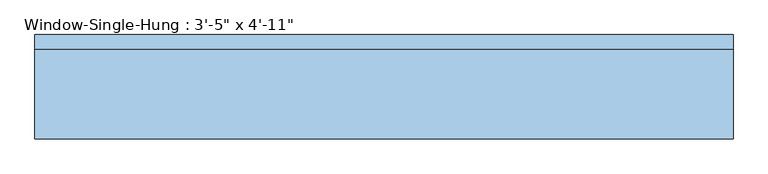
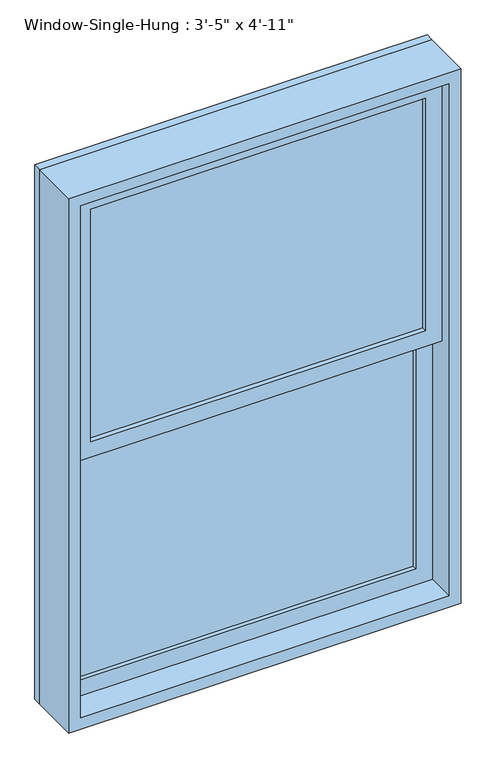
"""IFC4 building model written with IfcOpenShell, lengths in millimetres: window geometry."""

import ifcopenshell
import ifcopenshell.guid

model = None  # the IFC model being written
_history = None  # IfcOwnerHistory: only IFC2X3 demands one
_inside = {}  # id of a spatial element -> (the spatial element, [elements in it])
_under = {}  # id of a project, library or spatial element -> (it, [spatial elements below it])
_declared = {}  # id of a project -> (the project, [libraries it declares])
_typed = {}  # id of a type object -> (the type object, [elements of that type])
_made_of = {}  # id of a material, layer set ... -> (it, [elements and type objects made of it])


def new_model(schema):
    """Start an empty IFC model of exactly this schema.

    Asked for "IFC4X3", IfcOpenShell would pick the latest addendum, in which some entities
    have other attributes; the version numbers below select the first issue.
    IFC2X3 requires an IfcOwnerHistory on every rooted entity: one is made here for all.
    """
    global model, _history
    if schema == "IFC4X3":
        model = ifcopenshell.file(schema_version=(4, 3, 0, 0))
    else:
        model = ifcopenshell.file(schema=schema)
    _inside.clear()
    _under.clear()
    _declared.clear()
    _typed.clear()
    _made_of.clear()
    _history = None
    if model.schema == "IFC2X3":
        org = make("IfcOrganization", Name="unknown")
        user = make(
            "IfcPersonAndOrganization",
            ThePerson=make("IfcPerson", FamilyName="unknown"),
            TheOrganization=org,
        )
        app = make(
            "IfcApplication",
            ApplicationDeveloper=org,
            Version="unknown",
            ApplicationFullName="unknown",
            ApplicationIdentifier="unknown",
        )
        _history = make(
            "IfcOwnerHistory",
            OwningUser=user,
            OwningApplication=app,
            ChangeAction="ADDED",
            CreationDate=0,
        )
    return model


def make(cls, **values):
    """One entity of the class cls with the attributes given. An attribute that is None is left unset."""
    return model.create_entity(
        cls, **{name: value for name, value in values.items() if value is not None}
    )


def rooted(cls, **values):
    """An entity with a GlobalId (a new one), such as an element, a storey or a relation."""
    return make(cls, GlobalId=ifcopenshell.guid.new(), OwnerHistory=_history, **values)


def si_unit(unit_type, name, prefix=None):
    """IfcSIUnit, for example si_unit("LENGTHUNIT", "METRE", prefix="MILLI")."""
    return make("IfcSIUnit", UnitType=unit_type, Prefix=prefix, Name=name)


def assignment(units):
    """IfcUnitAssignment: the units of a project."""
    return None if units is None else make("IfcUnitAssignment", Units=units)


def point(xyz):
    """IfcCartesianPoint."""
    return None if xyz is None else make("IfcCartesianPoint", Coordinates=xyz)


def direction(xyz):
    """IfcDirection."""
    return None if xyz is None else make("IfcDirection", DirectionRatios=xyz)


def frame(location, z_axis=None, x_axis=None):
    """IfcAxis2Placement3D, a coordinate frame: its origin and axes. An axis left out is left unset."""
    return make(
        "IfcAxis2Placement3D",
        Location=point(location),
        Axis=direction(z_axis),
        RefDirection=direction(x_axis),
    )


def origin():
    """The frame at (0, 0, 0) with its axes left unset."""
    return frame((0.0, 0.0, 0.0))


def place(relative_to, where):
    """IfcLocalPlacement: puts the frame where relative to a parent placement (None: the world)."""
    return make(
        "IfcLocalPlacement", PlacementRelTo=relative_to, RelativePlacement=where
    )


def context(
    kind, dimensions, precision=None, world=None, true_north=None, identifier=None
):
    """IfcGeometricRepresentationContext, for example the 3D "Model" context."""
    return make(
        "IfcGeometricRepresentationContext",
        ContextIdentifier=identifier,
        ContextType=kind,
        CoordinateSpaceDimension=dimensions,
        Precision=precision,
        WorldCoordinateSystem=world,
        TrueNorth=true_north,
    )


def project(units=None, contexts=None):
    """IfcProject with its units and contexts."""
    return rooted(
        "IfcProject",
        Name="project",
        RepresentationContexts=contexts,
        UnitsInContext=assignment(units),
    )


def spatial(cls, under=None, at=None, **own):
    """A site, building, storey or space (cls), placed at a placement, below another one or the project."""
    s = rooted(cls, ObjectPlacement=at, **own)
    if under is not None:
        _under.setdefault(under.id(), (under, []))[1].append(s)
    return s


def polyline(points):
    """IfcPolyline through the points."""
    return make("IfcPolyline", Points=[point(p) for p in points])


def outline(outer, holes=None, kind="AREA"):
    """IfcArbitraryClosedProfileDef: a profile drawn as a closed curve; with holes, ...WithVoids."""
    if holes is None:
        return make("IfcArbitraryClosedProfileDef", ProfileType=kind, OuterCurve=outer)
    return make(
        "IfcArbitraryProfileDefWithVoids",
        ProfileType=kind,
        OuterCurve=outer,
        InnerCurves=holes,
    )


def extrude(swept, where, along, depth):
    """IfcExtrudedAreaSolid: the profile swept, set in the frame where, extruded along a direction by depth."""
    return make(
        "IfcExtrudedAreaSolid",
        SweptArea=swept,
        Position=where,
        ExtrudedDirection=direction(along),
        Depth=depth,
    )


def shape(context_of_items, identifier, shape_type, items):
    """IfcShapeRepresentation: the items that make up one representation, for example the "Body"."""
    return make(
        "IfcShapeRepresentation",
        ContextOfItems=context_of_items,
        RepresentationIdentifier=identifier,
        RepresentationType=shape_type,
        Items=items,
    )


def source(mapping_origin, context_of_items, identifier, shape_type, items):
    """IfcRepresentationMap: a shape defined once, which mapped items show again and again."""
    return make(
        "IfcRepresentationMap",
        MappingOrigin=mapping_origin,
        MappedRepresentation=shape(context_of_items, identifier, shape_type, items),
    )


def transform(
    local_origin,
    x_axis=None,
    y_axis=None,
    z_axis=None,
    scale=None,
    scale2=None,
    scale3=None,
    uniform=True,
):
    """IfcCartesianTransformationOperator3D, or its non-uniform kind. x_axis, y_axis, z_axis: its Axis1, 2, 3."""
    if uniform:
        return make(
            "IfcCartesianTransformationOperator3D",
            Axis1=direction(x_axis),
            Axis2=direction(y_axis),
            LocalOrigin=point(local_origin),
            Scale=scale,
            Axis3=direction(z_axis),
        )
    return make(
        "IfcCartesianTransformationOperator3DnonUniform",
        Axis1=direction(x_axis),
        Axis2=direction(y_axis),
        LocalOrigin=point(local_origin),
        Scale=scale,
        Axis3=direction(z_axis),
        Scale2=scale2,
        Scale3=scale3,
    )


def mapped(mapping_source, mapping_target):
    """IfcMappedItem: shows the shape of a source again, moved by a transform."""
    return make(
        "IfcMappedItem", MappingSource=mapping_source, MappingTarget=mapping_target
    )


def made_of(thing, what):
    """Note that an element or type object is made of a material, layer set ...; save() writes the relation."""
    if what is not None:
        _made_of.setdefault(what.id(), (what, []))[1].append(thing)
    return thing


def element(
    cls,
    number,
    at=None,
    inside=None,
    cuts=None,
    type_object=None,
    material=None,
    context=None,
    identifier="Body",
    shape_type=None,
    held_by="IfcProductDefinitionShape",
    body=None,
    shapes=None,
    **own,
):
    """One element of the class cls, such as IfcWall. Its Tag is "e" and its number.

    at: its placement. inside: the storey or other place that contains it. cuts: it is an
    opening in that element (IfcRelVoidsElement). A single representation is given by context,
    identifier, shape_type and body (its items); several are given by shapes. held_by: the class
    of the entity that holds the representations. save() writes the other relations.
    """
    e = rooted(cls, Tag="e%d" % number, ObjectPlacement=at, **own)
    if body is not None:
        shapes = [shape(context, identifier, shape_type, body)]
    if shapes is not None:
        e.Representation = make(held_by, Representations=shapes)
    if inside is not None:
        _inside.setdefault(inside.id(), (inside, []))[1].append(e)
    if cuts is not None:
        rooted(
            "IfcRelVoidsElement", RelatingBuildingElement=cuts, RelatedOpeningElement=e
        )
    if type_object is not None:
        _typed.setdefault(type_object.id(), (type_object, []))[1].append(e)
    return made_of(e, material)


def aggregate(whole, parts):
    """IfcRelAggregates: a whole, such as a stair, and the parts it consists of."""
    return rooted("IfcRelAggregates", RelatingObject=whole, RelatedObjects=parts)


def save(model, path):
    """Write the relations noted so far, then the file.

    IfcRelAggregates (storeys below a building ...), IfcRelContainedInSpatialStructure (elements
    in a storey), IfcRelDefinesByType, IfcRelAssociatesMaterial and IfcRelDeclares: one each for
    every whole, place, type object, material and project.
    """
    for whole, parts in _under.values():
        aggregate(whole, parts)
    for where, things in _inside.values():
        rooted(
            "IfcRelContainedInSpatialStructure",
            RelatedElements=things,
            RelatingStructure=where,
        )
    for kind, things in _typed.values():
        rooted("IfcRelDefinesByType", RelatedObjects=things, RelatingType=kind)
    for what, things in _made_of.values():
        rooted("IfcRelAssociatesMaterial", RelatedObjects=things, RelatingMaterial=what)
    for by, libraries in _declared.values():
        rooted("IfcRelDeclares", RelatingContext=by, RelatedDefinitions=libraries)
    model.write(path)


def window_d73c3647(model_context):
    return source(origin(), model_context, "Body", "SweptSolid", [
        extrude(outline(polyline([(444.5, 1.5875), (-444.5, 1.5875), (-444.5, 7.9375), (444.5, 7.9375), (444.5, 1.5875)])), frame((0.0, 0.0, 990.6), z_axis=(0.0, 0.0, 1.0), x_axis=(1.0, 0.0, 0.0)), (0.0, 0.0, 1.0), 650.875),
        extrude(outline(polyline([(-444.5, 14.2875), (-444.5, 20.6375), (444.5, 20.6375), (444.5, 14.2875), (-444.5, 14.2875)])), frame((0.0, 0.0, 990.6), z_axis=(0.0, 0.0, 1.0), x_axis=(1.0, 0.0, 0.0)), (0.0, 0.0, 1.0), 650.875),
        extrude(outline(polyline([(444.5, -42.8625), (-444.5, -42.8625), (-444.5, -36.5125), (444.5, -36.5125), (444.5, -42.8625)])), frame((0.0, 0.0, 1685.925), z_axis=(0.0, 0.0, 1.0), x_axis=(1.0, 0.0, 0.0)), (0.0, 0.0, 1.0), 650.875),
        extrude(outline(polyline([(-444.5, -30.1625), (-444.5, -23.8125), (444.5, -23.8125), (444.5, -30.1625), (-444.5, -30.1625)])), frame((0.0, 0.0, 1685.925), z_axis=(0.0, 0.0, 1.0), x_axis=(1.0, 0.0, 0.0)), (0.0, 0.0, 1.0), 650.875),
        extrude(outline(polyline([(1685.925, 488.95), (1685.925, -488.95), (946.15, -488.95), (946.15, 488.95), (1685.925, 488.95)]), holes=[polyline([(1641.475, -444.5), (1641.475, 444.5), (990.6, 444.5), (990.6, -444.5), (1641.475, -444.5)])]), frame((0.0, -11.1125, 0.0), z_axis=(0.0, 1.0, 0.0), x_axis=(0.0, 0.0, 1.0)), (0.0, 0.0, 1.0), 44.45),
        extrude(outline(polyline([(2381.25, 488.95), (2381.25, -488.95), (1641.475, -488.95), (1641.475, 488.95), (2381.25, 488.95)]), holes=[polyline([(2336.8, -444.5), (2336.8, 444.5), (1685.925, 444.5), (1685.925, -444.5), (2336.8, -444.5)])]), frame((0.0, -55.5625, 0.0), z_axis=(0.0, 1.0, 0.0), x_axis=(0.0, 0.0, 1.0)), (0.0, 0.0, 1.0), 44.45),
        extrude(outline(polyline([(2413.0, 520.7), (2413.0, -520.7), (914.4, -520.7), (914.4, 520.7), (2413.0, 520.7)]), holes=[polyline([(2381.25, -488.95), (2381.25, 488.95), (946.15, 488.95), (946.15, -488.95), (2381.25, -488.95)])]), frame((0.0, -87.3125, 0.0), z_axis=(0.0, 1.0, 0.0), x_axis=(0.0, 0.0, 1.0)), (0.0, 0.0, 1.0), 133.35),
        extrude(outline(polyline([(2413.0, 520.7), (2413.0, -520.7), (914.4, -520.7), (914.4, 520.7), (2413.0, 520.7)]), holes=[polyline([(2393.95, 501.65), (933.45, 501.65), (933.45, -501.65), (2393.95, -501.65), (2393.95, 501.65)])]), frame((0.0, 46.0375, 0.0), z_axis=(0.0, 1.0, 0.0), x_axis=(0.0, 0.0, 1.0)), (0.0, 0.0, 1.0), 22.225),
    ])


if __name__ == "__main__":
    model = new_model("IFC4")
    model_context = context("Model", 3, world=origin())
    ifc_project = project(units=[si_unit("LENGTHUNIT", "METRE", prefix="MILLI")], contexts=[model_context])
    site = spatial("IfcSite", under=ifc_project)
    building = spatial("IfcBuilding", under=site)
    placement = place(None, origin())
    window_shape = window_d73c3647(model_context)
    element("IfcWindow", 1, ObjectType="Window-Single-Hung : 3'-5\" x 4'-11\"", at=placement, inside=building, context=model_context, shape_type="MappedRepresentation", body=[
        mapped(window_shape, transform((0.0, 0.0, 0.0), x_axis=(1.0, 0.0, 0.0), y_axis=(0.0, 1.0, 0.0), z_axis=(0.0, 0.0, 1.0))),
    ])
    save(model, "model.ifc")

# Revit data of these elements
# Type "Window-Single-Hung : 3'-5\" x 4'-11\""
#   Type Mark = "21"
#   Fire Rating = "0.5h"
#   Construction Type Id = "DG-DR"
#   Assembly Code = "B2020100"
#   Analytic Construction = "Double glazing - domestic"
#   Wall Thickness [instance default] = 0' - 6"
#   Window Inset [instance default] = 0' - 0"
#   Visual Light Transmittance = 0.81
#   Thermal Resistance (R) = 0.319569 (m²·K)/W
#   Solar Heat Gain Coefficient = 0.76
#   Muntin Width = 2' - 11"
#   Muntin Height = 2' - 1 5/8"
#   Interior Wall Closure [instance default] = 0' - 1 1/2"
#   Rough Width = 3' - 5 1/2"
#   Rough Height = 4' - 11 1/2"
#   Frame Extension [instance default] = 0' - 1 1/4"
#   Exterior Wall Closure [instance default] = 0' - 0 1/2"
#   Extension Jamb [instance default] = 0' - 1 1/2"
#   Heat Transfer Coefficient (U) = 3.12929 W/(m²·K)
#   Height = 4' - 11"
#   Width = 3' - 5"
#   Top Muntin Visibility = yes
#   Indicator Visibility [instance default] = yes
#   Extension Jamb Visibility [instance default] = yes
#   Interior Trim Visibility [instance default] = yes
#   Exterior Trim Visibility [instance default] = yes
#   Bottom Muntin Visibility = yes
#   Muntin Pattern = Muntin Pattern_2x2 : Muntin Pattern_2x2
#   Interior Trim Material = Wood - Stained
#   Interior Trim = Trim-Window-Interior-Flat : Picture Frame
#   Exterior Trim Material = Clad - White
#   Exterior Trim = Trim-Window-Exterior-Flat : with Sill
#   Glass Panel Material = Glass
#   Exterior Frame Material = Clad - White
#   Interior Frame Material = Wood - Stained
#   Wall Closure = (empty or 0)
# Element 1 (IfcWindow, "Window-Single-Hung : 3'-5\" x 4'-11\"")
#   Wall Thickness = 0' - 5 3/8"
#   Extension Jamb = 0' - 0 7/8"
#   Materials on its faces: "Wood - Stained", "Glass", "Clad - White"
# Materials
#   "Wood - Stained": class "Wood", colour RGB 224 178 126, transparency 0, Cost = 0
#   "Clad - White": class "Wood", colour RGB 242 242 238, transparency 0, Cost = 0
#   "Glass": class "Glass", colour RGB 0 128 192, transparency 0.75, Description = "Soda Lime Glass", Cost = 0
